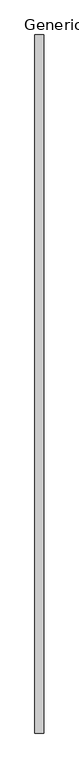
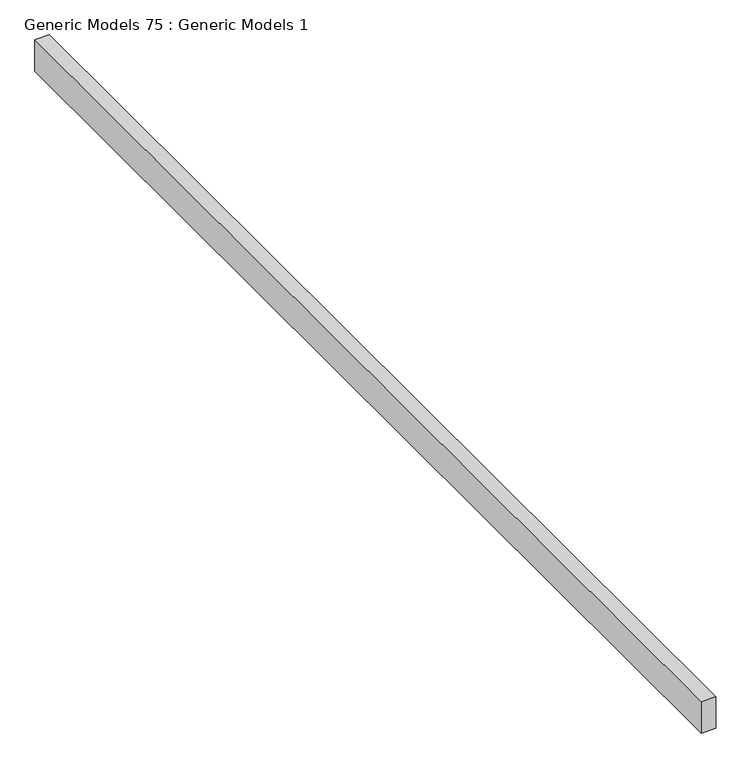
"""IFC4 building model written with IfcOpenShell, lengths in millimetres: proxy geometry, Generic Models 75 : Generic Models 1."""

import ifcopenshell
import ifcopenshell.guid

model = None  # the IFC model being written
_history = None  # IfcOwnerHistory: only IFC2X3 demands one
_inside = {}  # id of a spatial element -> (the spatial element, [elements in it])
_under = {}  # id of a project, library or spatial element -> (it, [spatial elements below it])
_declared = {}  # id of a project -> (the project, [libraries it declares])
_typed = {}  # id of a type object -> (the type object, [elements of that type])
_made_of = {}  # id of a material, layer set ... -> (it, [elements and type objects made of it])


def new_model(schema):
    """Start an empty IFC model of exactly this schema.

    Asked for "IFC4X3", IfcOpenShell would pick the latest addendum, in which some entities
    have other attributes; the version numbers below select the first issue.
    IFC2X3 requires an IfcOwnerHistory on every rooted entity: one is made here for all.
    """
    global model, _history
    if schema == "IFC4X3":
        model = ifcopenshell.file(schema_version=(4, 3, 0, 0))
    else:
        model = ifcopenshell.file(schema=schema)
    _inside.clear()
    _under.clear()
    _declared.clear()
    _typed.clear()
    _made_of.clear()
    _history = None
    if model.schema == "IFC2X3":
        org = make("IfcOrganization", Name="unknown")
        user = make(
            "IfcPersonAndOrganization",
            ThePerson=make("IfcPerson", FamilyName="unknown"),
            TheOrganization=org,
        )
        app = make(
            "IfcApplication",
            ApplicationDeveloper=org,
            Version="unknown",
            ApplicationFullName="unknown",
            ApplicationIdentifier="unknown",
        )
        _history = make(
            "IfcOwnerHistory",
            OwningUser=user,
            OwningApplication=app,
            ChangeAction="ADDED",
            CreationDate=0,
        )
    return model


def make(cls, **values):
    """One entity of the class cls with the attributes given. An attribute that is None is left unset."""
    return model.create_entity(
        cls, **{name: value for name, value in values.items() if value is not None}
    )


def rooted(cls, **values):
    """An entity with a GlobalId (a new one), such as an element, a storey or a relation."""
    return make(cls, GlobalId=ifcopenshell.guid.new(), OwnerHistory=_history, **values)


def si_unit(unit_type, name, prefix=None):
    """IfcSIUnit, for example si_unit("LENGTHUNIT", "METRE", prefix="MILLI")."""
    return make("IfcSIUnit", UnitType=unit_type, Prefix=prefix, Name=name)


def assignment(units):
    """IfcUnitAssignment: the units of a project."""
    return None if units is None else make("IfcUnitAssignment", Units=units)


def point(xyz):
    """IfcCartesianPoint."""
    return None if xyz is None else make("IfcCartesianPoint", Coordinates=xyz)


def direction(xyz):
    """IfcDirection."""
    return None if xyz is None else make("IfcDirection", DirectionRatios=xyz)


def frame(location, z_axis=None, x_axis=None):
    """IfcAxis2Placement3D, a coordinate frame: its origin and axes. An axis left out is left unset."""
    return make(
        "IfcAxis2Placement3D",
        Location=point(location),
        Axis=direction(z_axis),
        RefDirection=direction(x_axis),
    )


def origin():
    """The frame at (0, 0, 0) with its axes left unset."""
    return frame((0.0, 0.0, 0.0))


def place(relative_to, where):
    """IfcLocalPlacement: puts the frame where relative to a parent placement (None: the world)."""
    return make(
        "IfcLocalPlacement", PlacementRelTo=relative_to, RelativePlacement=where
    )


def context(
    kind, dimensions, precision=None, world=None, true_north=None, identifier=None
):
    """IfcGeometricRepresentationContext, for example the 3D "Model" context."""
    return make(
        "IfcGeometricRepresentationContext",
        ContextIdentifier=identifier,
        ContextType=kind,
        CoordinateSpaceDimension=dimensions,
        Precision=precision,
        WorldCoordinateSystem=world,
        TrueNorth=true_north,
    )


def project(units=None, contexts=None):
    """IfcProject with its units and contexts."""
    return rooted(
        "IfcProject",
        Name="project",
        RepresentationContexts=contexts,
        UnitsInContext=assignment(units),
    )


def spatial(cls, under=None, at=None, **own):
    """A site, building, storey or space (cls), placed at a placement, below another one or the project."""
    s = rooted(cls, ObjectPlacement=at, **own)
    if under is not None:
        _under.setdefault(under.id(), (under, []))[1].append(s)
    return s


def polyline(points):
    """IfcPolyline through the points."""
    return make("IfcPolyline", Points=[point(p) for p in points])


def outline(outer, holes=None, kind="AREA"):
    """IfcArbitraryClosedProfileDef: a profile drawn as a closed curve; with holes, ...WithVoids."""
    if holes is None:
        return make("IfcArbitraryClosedProfileDef", ProfileType=kind, OuterCurve=outer)
    return make(
        "IfcArbitraryProfileDefWithVoids",
        ProfileType=kind,
        OuterCurve=outer,
        InnerCurves=holes,
    )


def extrude(swept, where, along, depth):
    """IfcExtrudedAreaSolid: the profile swept, set in the frame where, extruded along a direction by depth."""
    return make(
        "IfcExtrudedAreaSolid",
        SweptArea=swept,
        Position=where,
        ExtrudedDirection=direction(along),
        Depth=depth,
    )


def shape(context_of_items, identifier, shape_type, items):
    """IfcShapeRepresentation: the items that make up one representation, for example the "Body"."""
    return make(
        "IfcShapeRepresentation",
        ContextOfItems=context_of_items,
        RepresentationIdentifier=identifier,
        RepresentationType=shape_type,
        Items=items,
    )


def source(mapping_origin, context_of_items, identifier, shape_type, items):
    """IfcRepresentationMap: a shape defined once, which mapped items show again and again."""
    return make(
        "IfcRepresentationMap",
        MappingOrigin=mapping_origin,
        MappedRepresentation=shape(context_of_items, identifier, shape_type, items),
    )


def transform(
    local_origin,
    x_axis=None,
    y_axis=None,
    z_axis=None,
    scale=None,
    scale2=None,
    scale3=None,
    uniform=True,
):
    """IfcCartesianTransformationOperator3D, or its non-uniform kind. x_axis, y_axis, z_axis: its Axis1, 2, 3."""
    if uniform:
        return make(
            "IfcCartesianTransformationOperator3D",
            Axis1=direction(x_axis),
            Axis2=direction(y_axis),
            LocalOrigin=point(local_origin),
            Scale=scale,
            Axis3=direction(z_axis),
        )
    return make(
        "IfcCartesianTransformationOperator3DnonUniform",
        Axis1=direction(x_axis),
        Axis2=direction(y_axis),
        LocalOrigin=point(local_origin),
        Scale=scale,
        Axis3=direction(z_axis),
        Scale2=scale2,
        Scale3=scale3,
    )


def mapped(mapping_source, mapping_target):
    """IfcMappedItem: shows the shape of a source again, moved by a transform."""
    return make(
        "IfcMappedItem", MappingSource=mapping_source, MappingTarget=mapping_target
    )


def made_of(thing, what):
    """Note that an element or type object is made of a material, layer set ...; save() writes the relation."""
    if what is not None:
        _made_of.setdefault(what.id(), (what, []))[1].append(thing)
    return thing


def element(
    cls,
    number,
    at=None,
    inside=None,
    cuts=None,
    type_object=None,
    material=None,
    context=None,
    identifier="Body",
    shape_type=None,
    held_by="IfcProductDefinitionShape",
    body=None,
    shapes=None,
    **own,
):
    """One element of the class cls, such as IfcWall. Its Tag is "e" and its number.

    at: its placement. inside: the storey or other place that contains it. cuts: it is an
    opening in that element (IfcRelVoidsElement). A single representation is given by context,
    identifier, shape_type and body (its items); several are given by shapes. held_by: the class
    of the entity that holds the representations. save() writes the other relations.
    """
    e = rooted(cls, Tag="e%d" % number, ObjectPlacement=at, **own)
    if body is not None:
        shapes = [shape(context, identifier, shape_type, body)]
    if shapes is not None:
        e.Representation = make(held_by, Representations=shapes)
    if inside is not None:
        _inside.setdefault(inside.id(), (inside, []))[1].append(e)
    if cuts is not None:
        rooted(
            "IfcRelVoidsElement", RelatingBuildingElement=cuts, RelatedOpeningElement=e
        )
    if type_object is not None:
        _typed.setdefault(type_object.id(), (type_object, []))[1].append(e)
    return made_of(e, material)


def aggregate(whole, parts):
    """IfcRelAggregates: a whole, such as a stair, and the parts it consists of."""
    return rooted("IfcRelAggregates", RelatingObject=whole, RelatedObjects=parts)


def save(model, path):
    """Write the relations noted so far, then the file.

    IfcRelAggregates (storeys below a building ...), IfcRelContainedInSpatialStructure (elements
    in a storey), IfcRelDefinesByType, IfcRelAssociatesMaterial and IfcRelDeclares: one each for
    every whole, place, type object, material and project.
    """
    for whole, parts in _under.values():
        aggregate(whole, parts)
    for where, things in _inside.values():
        rooted(
            "IfcRelContainedInSpatialStructure",
            RelatedElements=things,
            RelatingStructure=where,
        )
    for kind, things in _typed.values():
        rooted("IfcRelDefinesByType", RelatedObjects=things, RelatingType=kind)
    for what, things in _made_of.values():
        rooted("IfcRelAssociatesMaterial", RelatedObjects=things, RelatingMaterial=what)
    for by, libraries in _declared.values():
        rooted("IfcRelDeclares", RelatingContext=by, RelatedDefinitions=libraries)
    model.write(path)


def generic_models_75_generic_models_1_f7ba8b09(model_context):
    return source(origin(), model_context, "Body", "SweptSolid", [
        extrude(outline(polyline([(-8344.0736296, 7054.2769662), (-8166.2736296, 7054.2769662), (-8166.2736296, -7068.1230338), (-8344.0736296, -7068.1230338), (-8344.0736296, 7054.2769662)])), frame((0.0, 0.0, 126345.696), z_axis=(0.0, 0.0, 1.0), x_axis=(1.0, 0.0, 0.0)), (0.0, 0.0, 1.0), 406.4),
    ])


if __name__ == "__main__":
    model = new_model("IFC4")
    model_context = context("Model", 3, world=origin())
    ifc_project = project(units=[si_unit("LENGTHUNIT", "METRE", prefix="MILLI")], contexts=[model_context])
    site = spatial("IfcSite", under=ifc_project)
    building = spatial("IfcBuilding", under=site)
    placement = place(None, origin())
    generic_models_75_generic_models_1_shape = generic_models_75_generic_models_1_f7ba8b09(model_context)
    element("IfcBuildingElementProxy", 1, Name="Generic Models 75 : Generic Models 1", ObjectType="Generic Models 75 : Generic Models 1", at=placement, inside=building, context=model_context, shape_type="MappedRepresentation", body=[
        mapped(generic_models_75_generic_models_1_shape, transform((0.0, 0.0, 0.0), x_axis=(1.0, 0.0, 0.0), y_axis=(0.0, 1.0, 0.0), z_axis=(0.0, 0.0, 1.0))),
    ])
    save(model, "model.ifc")

# Revit data of these elements
# Element 1 (IfcBuildingElementProxy, "Generic Models 75 : Generic Models 1")
#   Materials on its faces: "_STRUCTURAL MEMBER (SEE STRUCT. DWGS)"
# Materials
#   "_STRUCTURAL MEMBER (SEE STRUCT. DWGS)": class "Generic", colour RGB 209 182 141, transparency 0, Cost = 0
